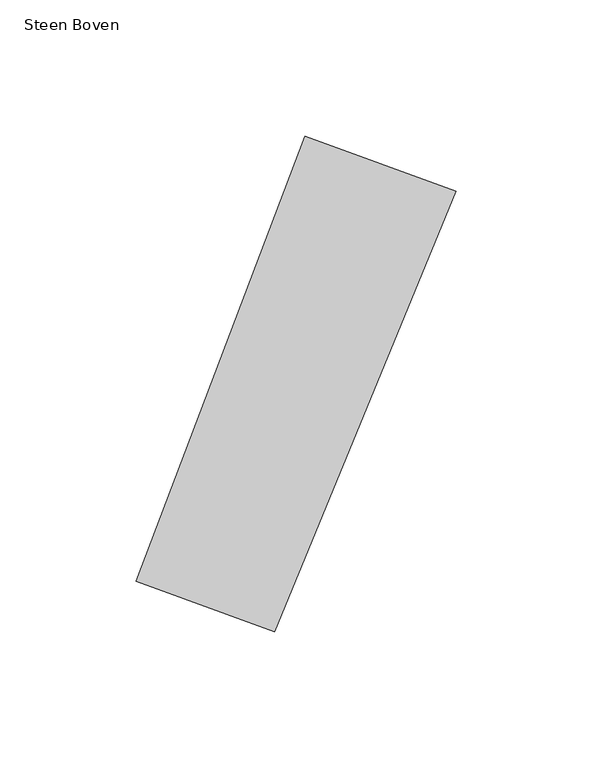
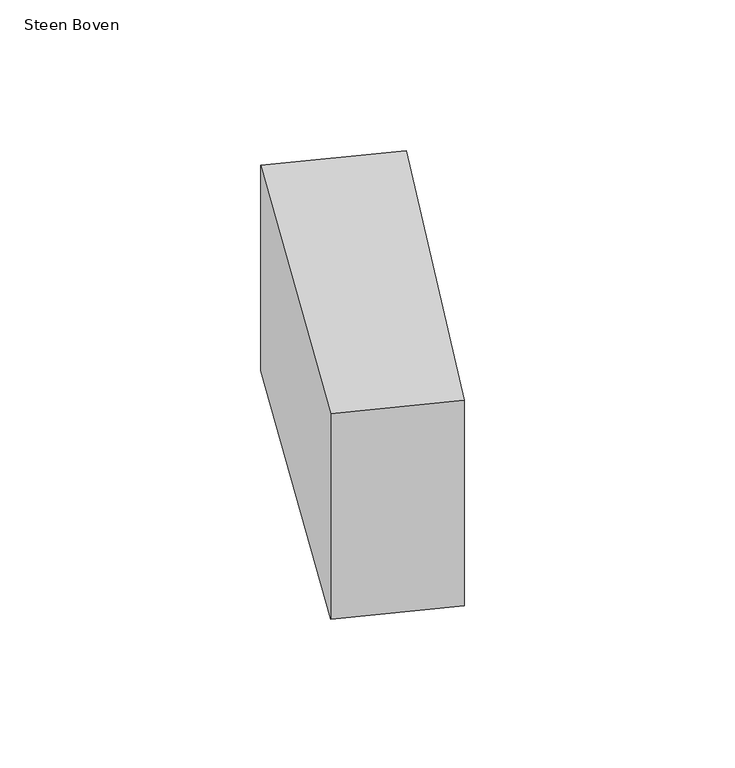
"""IFC4 building model written with IfcOpenShell, lengths in millimetres: proxy geometry, 00_GMA_steen_versie_4 : Steen Boven."""

from ifc_helpers import new_model, si_unit, origin, origin_with_axes, place, context, project, spatial, polyline, outline, extrude, source, transform, mapped, element, save


def steen_boven_5acc6e9e(model_context):
    return source(origin(), model_context, "Body", "SweptSolid", [
        extrude(outline(polyline([(135.1658053, 153.5946355), (68.4493406, -8.3551905), (17.5840745, 10.1818493), (79.7634128, 173.7814411), (135.1658053, 153.5946355)])), origin_with_axes(), (0.0, 0.0, 1.0), 100.0),
    ])


if __name__ == "__main__":
    model = new_model("IFC4")
    model_context = context("Model", 3, world=origin())
    ifc_project = project(units=[si_unit("LENGTHUNIT", "METRE", prefix="MILLI")], contexts=[model_context])
    site = spatial("IfcSite", under=ifc_project)
    building = spatial("IfcBuilding", under=site)
    placement = place(None, origin())
    steen_boven_shape = steen_boven_5acc6e9e(model_context)
    element("IfcBuildingElementProxy", 1, Name="00_GMA_steen_versie_4 : Steen Boven", ObjectType="00_GMA_steen_versie_4 : Steen Boven", at=placement, inside=building, context=model_context, shape_type="MappedRepresentation", body=[
        mapped(steen_boven_shape, transform((0.0, 0.0, 0.0), x_axis=(1.0, 0.0, 0.0), y_axis=(0.0, 1.0, 0.0), z_axis=(0.0, 0.0, 1.0))),
    ])
    save(model, "model.ifc")

# Revit data of these elements
# Type "00_GMA_steen_versie_4 : Steen Boven"
#   StootVoegHalfBoven [instance default] = 5 mm
#   StootVoegHalf [instance default] = 5 mm
#   StootVoegBreedteOnder = 10 mm
#   StootVoegBreedteBoven = 10 mm
#   Steendikte = 100 mm
#   LintVoegOnderHalf = 5 mm
#   LintVoegOnder = 10 mm
#   LintVoegBovenHalf = 0 mm
#   LintVoegBoven = 0 mm
#   materiaal = none
#   MateriaalVoeg = none
#   Default Elevation = 0
